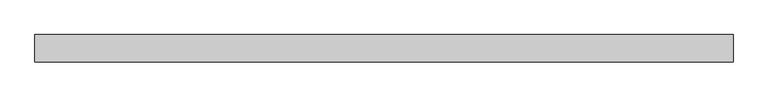
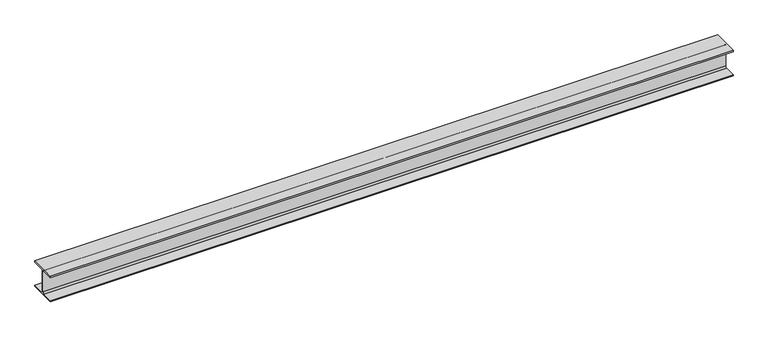
"""IFC4 building model written with IfcOpenShell, lengths in millimetres: beam geometry, 0912_Steel Framing_H-KSD3502 : H_SB_ASB_H-300x300x10x15."""

from ifc_helpers import new_model, si_unit, point, frame, frame_2d, origin, place, context, project, spatial, polyline, circle_curve, trimmed, segment, composite_curve, outline, extrude, source, transform, mapped, element, save


def beam_79ec66e8(model_context):
    return source(origin(), model_context, "Body", "SweptSolid", [
        extrude(outline(composite_curve([segment(polyline([(150.0, -135.0), (150.0, -150.0), (-150.0, -150.0), (-150.0, -135.0), (-23.0, -135.0)]), True, "CONTINUOUS"), segment(trimmed(circle_curve(frame_2d((-23.0, -117.0)), 18.0), [point((-23.0, -135.0))], [point((-5.0, -117.0))], True, "CARTESIAN"), True, "CONTINUOUS"), segment(polyline([(-5.0, -117.0), (-5.0, 117.0)]), True, "CONTINUOUS"), segment(trimmed(circle_curve(frame_2d((-23.0, 117.0)), 18.0), [point((-5.0, 117.0))], [point((-23.0, 135.0))], True, "CARTESIAN"), True, "CONTINUOUS"), segment(polyline([(-23.0, 135.0), (-150.0, 135.0), (-150.0, 150.0), (150.0, 150.0), (150.0, 135.0), (23.0, 135.0)]), True, "CONTINUOUS"), segment(trimmed(circle_curve(frame_2d((23.0, 117.0)), 18.0), [point((23.0, 135.0))], [point((5.0, 117.0))], True, "CARTESIAN"), True, "CONTINUOUS"), segment(polyline([(5.0, 117.0), (5.0, -117.0)]), True, "CONTINUOUS"), segment(trimmed(circle_curve(frame_2d((23.0, -117.0)), 18.0), [point((5.0, -117.0))], [point((23.0, -135.0))], True, "CARTESIAN"), True, "CONTINUOUS"), segment(polyline([(23.0, -135.0), (150.0, -135.0)]), True, "CONTINUOUS")], self_intersect=False)), frame((-3836.5021141, 0.0, 0.0), z_axis=(1.0, 0.0, 0.0), x_axis=(0.0, 1.0, 0.0)), (0.0, 0.0, 1.0), 7604.5653228),
    ])


if __name__ == "__main__":
    model = new_model("IFC4")
    model_context = context("Model", 3, world=origin())
    ifc_project = project(units=[si_unit("LENGTHUNIT", "METRE", prefix="MILLI")], contexts=[model_context])
    site = spatial("IfcSite", under=ifc_project)
    building = spatial("IfcBuilding", under=site)
    placement = place(None, origin())
    beam_shape = beam_79ec66e8(model_context)
    element("IfcBeam", 1, ObjectType="0912_Steel Framing_H-KSD3502 : H_SB_ASB_H-300x300x10x15", at=placement, inside=building, context=model_context, shape_type="MappedRepresentation", body=[
        mapped(beam_shape, transform((0.0, 0.0, 0.0), x_axis=(1.0, 0.0, 0.0), y_axis=(0.0, 1.0, 0.0), z_axis=(0.0, 0.0, 1.0))),
    ])
    save(model, "model.ifc")

# Revit data of these elements
# Type "0912_Steel Framing_H-KSD3502 : H_SB_ASB_H-300x300x10x15"
#   H_WM Code_1 = "S01AA001-00001 | Main Steel Structure Fabrication Work | Shelter/Building | Heavy Steel - Standard (Weight≥90KG/M) | Material: (   )"
#   H_WM Code_2 = "S03AA027-00001 | Main Steel Structure Erection Work | Shelter/Building | Heavy Steel (Weight≥90KG/M) | Material: (   )"
#   H_WM Code_3 = "S01AA010-00001 | Main Steel Structure Fabrication Work | Shelter/Building | Steel Painting/Coating | for Non-Fireproofed Steel Surface, Surface Preparation, Primer, Second & Final Coat | Material: (   )"
#   H_Q'ty Cal Type Tag = "SB-Q2"
#   Width = 30.0 cm
#   Web Thickness = 1.0 cm
#   Web Fillet = 1.8 cm
#   Warping Constant = 1370000.0 cm⁶
#   W = 0
#   Torsional Moment of Inertia = 77.00 cm⁴
#   Section Area = 119.8 cm²
#   Plastic Modulus weak axis = 684.0 cm³
#   Plastic Modulus strong axis = 1500.0 cm³
#   Perimeter = 1.75 m²/m
#   Nominal Weight = 94.00 kgf/m
#   Moment of Inertia weak axis = 6750.00 cm⁴
#   Moment of Inertia strong axis = 20400.00 cm⁴
#   Height = 30.0 cm
#   Flange Thickness = 1.5 cm
#   Elastic Modulus weak axis = 450.0 cm³
#   Elastic Modulus strong axis = 1360.0 cm³
#   Centroid Vertical = 15.0 cm
#   Centroid Horizontal = 15.0 cm
#   Ix = 204000000
#   Length [instance default] = 1.5240 m
#   Zx = 1500000
#   b = 0.3000 m
#   h = 0.3000 m
#   r = 0.0180 m
#   s = 0.0100 m
#   t = 0.0150 m
#   A = 0.01198 m²
#   Structural Material [instance default] = Steel, 45-345
#   Assembly Code = ""
# Element 1 (IfcBeam, "0912_Steel Framing_H-KSD3502 : H_SB_ASB_H-300x300x10x15")
#   Structural Material = none
# Materials
#   "Steel, 45-345": class "Metal", colour RGB 189 187 185, transparency 0, Description = "Steel 345 MPa", Cost = 0
